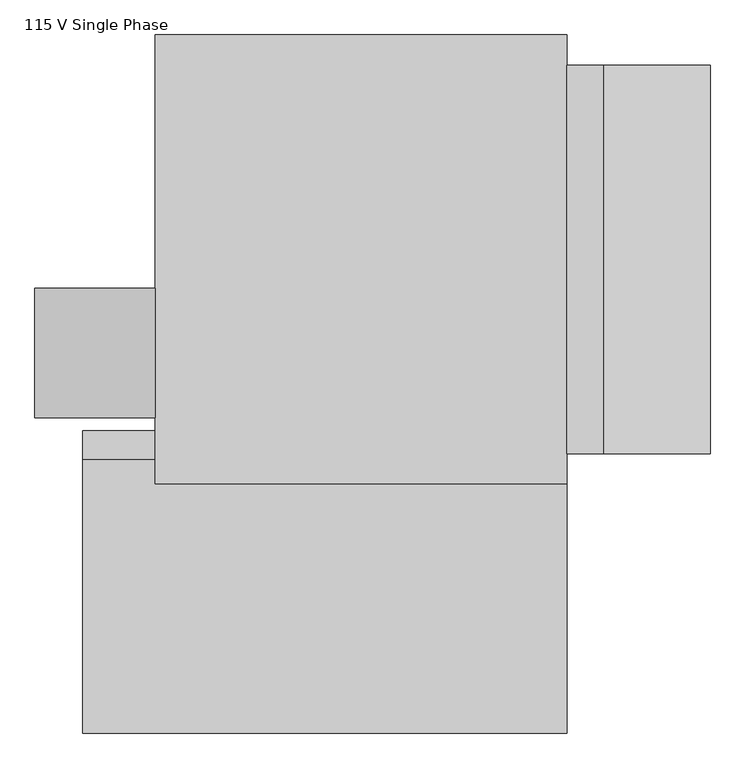
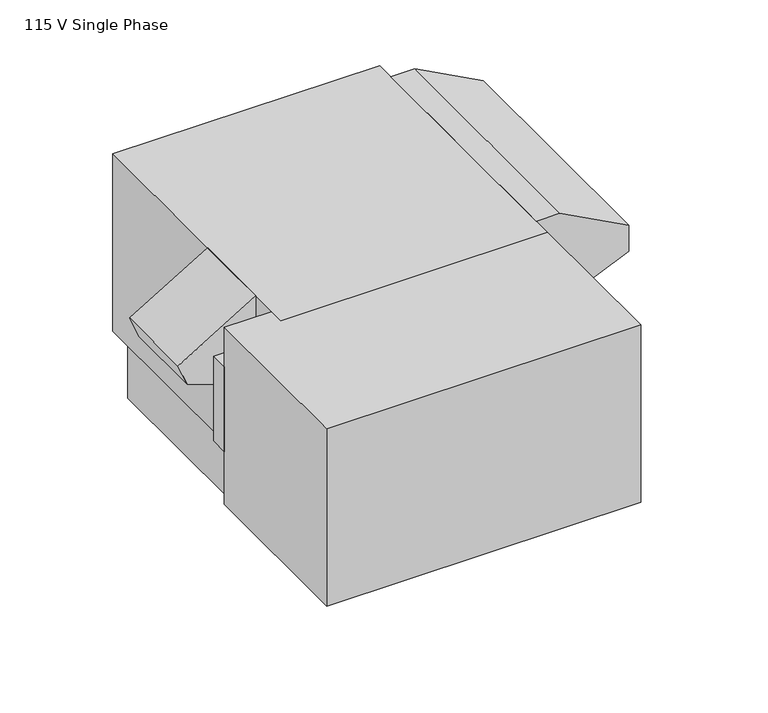
"""IFC4 building model written with IfcOpenShell, lengths in millimetres: proxy geometry, he3xrtf : 115 V Single Phase."""

from ifc_helpers import new_model, si_unit, frame, origin, place, context, project, spatial, polyline, outline, extrude, faceted_brep, source, transform, mapped, element, save


def proxy_115_v_single_phase_5f010b2a(model_context):
    return source(origin(), model_context, "Body", "SolidModel", [
        extrude(outline(polyline([(1377.95, 727.075), (807.0234515, 727.075), (1028.2003796, 1231.9), (1178.2391959, 1231.9), (1377.95, 857.25), (1377.95, 727.075)])), frame((0.0, -685.8, 0.0), z_axis=(0.0, 1.0, 0.0), x_axis=(0.0, 0.0, 1.0)), (0.0, 0.0, 1.0), 1371.6),
        extrude(outline(polyline([(870.6269912, -727.075), (1377.95, -727.075), (1123.1977683, -1152.525), (1000.019549, -1102.8582739), (870.6269912, -727.075)])), frame((0.0, -558.8, 0.0), z_axis=(0.0, 1.0, 0.0), x_axis=(0.0, 0.0, 1.0)), (0.0, 0.0, 1.0), 457.2),
        faceted_brep([(727.075, 792.1625, 1377.95), (-727.075, 792.1625, 1377.95), (-727.075, -792.1625, 1377.95), (727.075, -792.1625, 1377.95), (727.075, 792.1625, 355.6), (727.075, -792.1625, 355.6), (-727.075, -792.1625, 355.6), (-727.075, 792.1625, 355.6), (687.3875, 719.1375, 355.6), (-687.3875, 719.1375, 355.6), (-687.3875, -719.1375, 355.6), (687.3875, -719.1375, 355.6), (-727.075, -604.785477, 1149.35), (-727.075, -706.385477, 1149.35), (-727.075, -706.385477, 660.4), (-727.075, -604.785477, 660.4), (727.075, -404.8125, 790.575), (727.075, 458.7875, 790.575), (727.075, 458.7875, 485.775), (727.075, -404.8125, 485.775), (687.3875, 719.1375, 0.0), (687.3875, -719.1375, 0.0), (-687.3875, -719.1375, 0.0), (-687.3875, 719.1375, 0.0), (752.475, 458.7875, 790.575), (752.475, -404.8125, 790.575), (752.475, -404.8125, 485.775), (752.475, 458.7875, 485.775), (-984.25, -706.385477, 1149.35), (-984.25, -604.785477, 1149.35), (-984.25, -604.785477, 660.4), (-984.25, -706.385477, 660.4)], [[[0, 1, 2, 3]], [[4, 5, 6, 7], [8, 9, 10, 11]], [[1, 0, 4, 7]], [[2, 1, 7, 6], [12, 13, 14, 15]], [[3, 2, 6, 5]], [[0, 3, 5, 4], [16, 17, 18, 19]], [[20, 21, 22, 23]], [[20, 23, 9, 8]], [[23, 22, 10, 9]], [[22, 21, 11, 10]], [[21, 20, 8, 11]], [[24, 25, 26, 27]], [[25, 24, 17, 16]], [[26, 25, 16, 19]], [[27, 26, 19, 18]], [[24, 27, 18, 17]], [[28, 29, 30, 31]], [[29, 28, 13, 12]], [[30, 29, 12, 15]], [[31, 30, 15, 14]], [[28, 31, 14, 13]]]),
        extrude(outline(polyline([(727.075, -1671.6375), (-984.25, -1671.6375), (-984.25, -706.385477), (-727.075, -706.385477), (-727.075, -792.1625), (727.075, -792.1625), (727.075, -1671.6375)])), frame((0.0, 0.0, 355.6), z_axis=(0.0, 0.0, 1.0), x_axis=(1.0, 0.0, 0.0)), (0.0, 0.0, 1.0), 1022.35),
    ])


if __name__ == "__main__":
    model = new_model("IFC4")
    model_context = context("Model", 3, world=origin())
    ifc_project = project(units=[si_unit("LENGTHUNIT", "METRE", prefix="MILLI")], contexts=[model_context])
    site = spatial("IfcSite", under=ifc_project)
    building = spatial("IfcBuilding", under=site)
    placement = place(None, origin())
    proxy_115_v_single_phase_shape = proxy_115_v_single_phase_5f010b2a(model_context)
    element("IfcBuildingElementProxy", 1, Name="he3xrtf : 115 V Single Phase", ObjectType="he3xrtf : 115 V Single Phase", at=placement, inside=building, context=model_context, shape_type="MappedRepresentation", body=[
        mapped(proxy_115_v_single_phase_shape, transform((0.0, 0.0, 0.0), x_axis=(1.0, 0.0, 0.0), y_axis=(0.0, 1.0, 0.0), z_axis=(0.0, 0.0, 1.0))),
    ])
    save(model, "model.ifc")

# Revit data of these elements
# Type "he3xrtf : 115 V Single Phase"
#   URL = "http://www.renewaire.com/_assets/files/SubmittalForms/HE3XRTSubmittal.pdf"
#   Model = "HE3XRTF"
#   Manufacturer = "RenewAire"
#   Weight Scheduled [instance default] = 726
#   Voltage Workaround = 115
#   Voltage Scheduled = 115 V
#   Voltage = 115 V
#   VoltAmps Workaround [instance default] = 0
#   VoltAmps [instance default] = 0 VA
#   Total FLA [instance default] = 0
#   Supply Motor RPM Scheduled [instance default] = 0
#   Supply Motor RPM [instance default] = 0
#   Supply Motor HP Scheduled [instance default] = 0
#   Supply Motor HP [instance default] = 0
#   Supply Motor FLA [instance default] = 0
#   Supply Motor Count Scheduled [instance default] = 1
#   Supply Motor Count [instance default] = 1
#   Supply Motor BHP [instance default] = 0
#   Supply ESP Scheduled [instance default] = 0
#   Supply ESP [instance default] = 0
#   Supply CFM Scheduled [instance default] = 0 CFM
#   Supply CFM [instance default] = 0 CFM
#   Supply Air Winter RH Scheduled [instance default] = 0
#   Supply Air Winter DB Scheduled [instance default] = 0
#   Supply Air Summer RH Scheduled [instance default] = 0
#   Supply Air Summer DB Scheduled [instance default] = 0
#   Phase Scheduled = 1
#   Phase = 1
#   Outside Air Winter RH Scheduled [instance default] = 0
#   Outside Air Winter DB Scheduled [instance default] = 0
#   Outside Air Summer RH Scheduled [instance default] = 0
#   Outside Air Summer DB Scheduled [instance default] = 0
#   MOCP Scheduled [instance default] = 0
#   MOCP [instance default] = 0
#   MCA Scheduled [instance default] = 0
#   MCA [instance default] = 0
#   FLA Scheduled [instance default] = 0
#   Exhaust RH Scheduled [instance default] = 0
#   Exhaust Motor RPM Scheduled [instance default] = 0
#   Exhaust Motor RPM [instance default] = 0
#   Exhaust Motor HP Scheduled [instance default] = 0
#   Exhaust Motor HP [instance default] = 0
#   Exhaust Motor FLA [instance default] = 0
#   Exhaust Motor Count Scheduled [instance default] = 1
#   Exhaust Motor Count [instance default] = 1
#   Exhaust Motor BHP [instance default] = 0
#   Exhaust ESP Scheduled [instance default] = 0
#   Exhaust ESP [instance default] = 0
#   Exhaust DB Scheduled [instance default] = 0
#   Exhaust CFM Scheduled [instance default] = 0 CFM
#   Exhaust CFM [instance default] = 0 CFM
#   Enthalpy Effect Winter Scheduled [instance default] = 0
#   Enthalpy Effect Summer Scheduled [instance default] = 0
#   VFD [instance default] = no
#   Number of Poles = 1
#   Material = RTU
# Element 1 (IfcBuildingElementProxy, "he3xrtf : 115 V Single Phase")
#   Materials on its faces: "RTU", "Clearance Zone"
# Materials
#   "RTU": class "Miscellaneous", colour RGB 104 104 104, transparency 0, Cost = 0
#   "Clearance Zone": class "Miscellaneous", colour RGB 255 0 0, transparency 0.8
